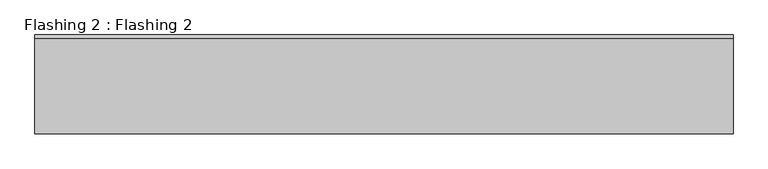
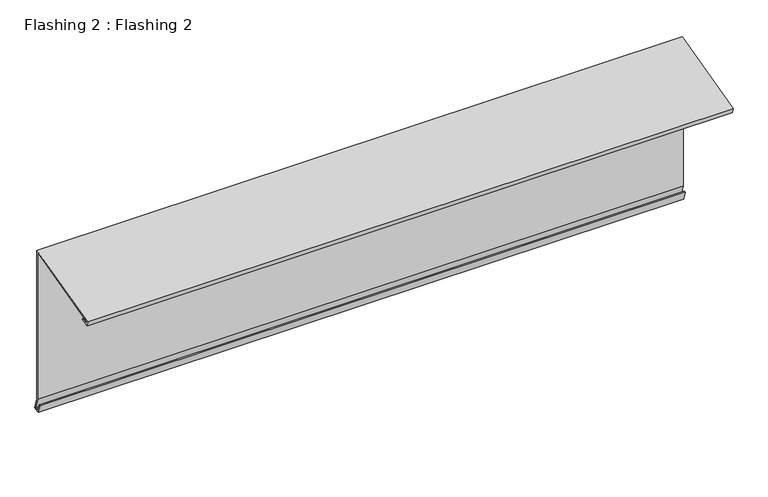
"""IFC4 building model written with IfcOpenShell, lengths in millimetres: proxy geometry, Flashing 2 : Flashing 2."""

from ifc_helpers import new_model, si_unit, frame, origin, place, context, project, spatial, polyline, outline, extrude, source, transform, mapped, element, save


def flashing_2_flashing_2_086f2f6e(model_context):
    return source(origin(), model_context, "Body", "SweptSolid", [
        extrude(outline(polyline([(10550.3613281, 43920.3046875), (10546.9589844, 43935.2734375), (10819.5097656, 44004.90625), (10819.5097656, 43518.7539063), (10830.6904297, 43482.3320313), (10813.1210937, 43476.9648438), (10804.5996094, 43504.4882813), (10808.4206617, 43505.6713107), (10815.7635636, 43481.9545626), (10825.6911014, 43484.9872871), (10815.5097656, 43518.1537731), (10815.5097656, 43999.7558251), (10551.7227627, 43932.3620321), (10553.3654045, 43925.1351625), (10575.0634961, 43930.3201524), (10575.9931641, 43926.4296875), (10550.3613281, 43920.3046875)])), frame((3694.0383192, 0.0, 0.0), z_axis=(1.0, 0.0, 0.0), x_axis=(0.0, 1.0, 0.0)), (0.0, 0.0, 1.0), 2000.25),
    ])


if __name__ == "__main__":
    model = new_model("IFC4")
    model_context = context("Model", 3, world=origin())
    ifc_project = project(units=[si_unit("LENGTHUNIT", "METRE", prefix="MILLI")], contexts=[model_context])
    site = spatial("IfcSite", under=ifc_project)
    building = spatial("IfcBuilding", under=site)
    placement = place(None, origin())
    flashing_2_flashing_2_shape = flashing_2_flashing_2_086f2f6e(model_context)
    element("IfcBuildingElementProxy", 1, Name="Flashing 2 : Flashing 2", ObjectType="Flashing 2 : Flashing 2", at=placement, inside=building, context=model_context, shape_type="MappedRepresentation", body=[
        mapped(flashing_2_flashing_2_shape, transform((0.0, 0.0, 0.0), x_axis=(1.0, 0.0, 0.0), y_axis=(0.0, 1.0, 0.0), z_axis=(0.0, 0.0, 1.0))),
    ])
    save(model, "model.ifc")

# Revit data of these elements
# Type "Flashing 2 : Flashing 2"
#   NameOverride = "Flashing"
# Element 1 (IfcBuildingElementProxy, "Flashing 2 : Flashing 2")
#   Materials on its faces: "HIGH EAVE FLASHING"
# Materials
#   "HIGH EAVE FLASHING": class "Unassigned", colour RGB 128 128 128, transparency 0
